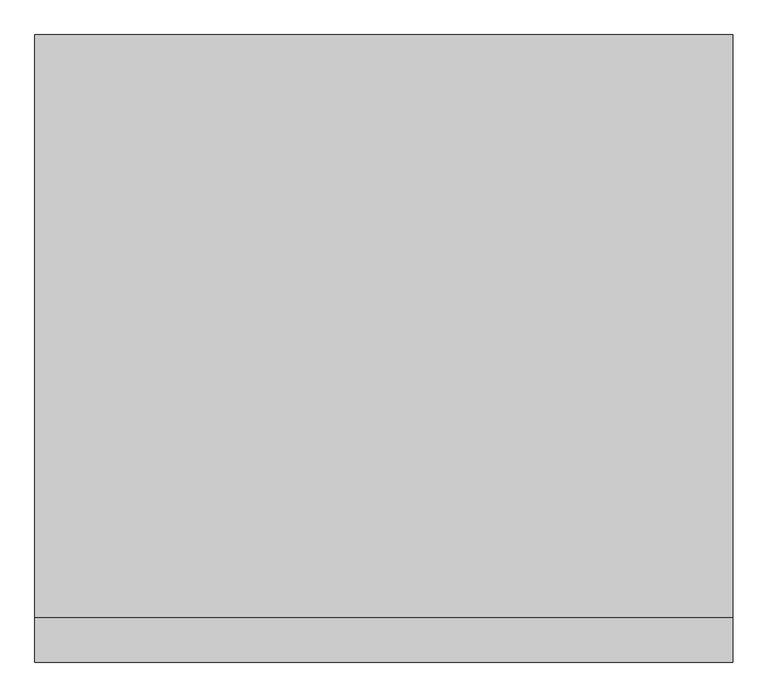
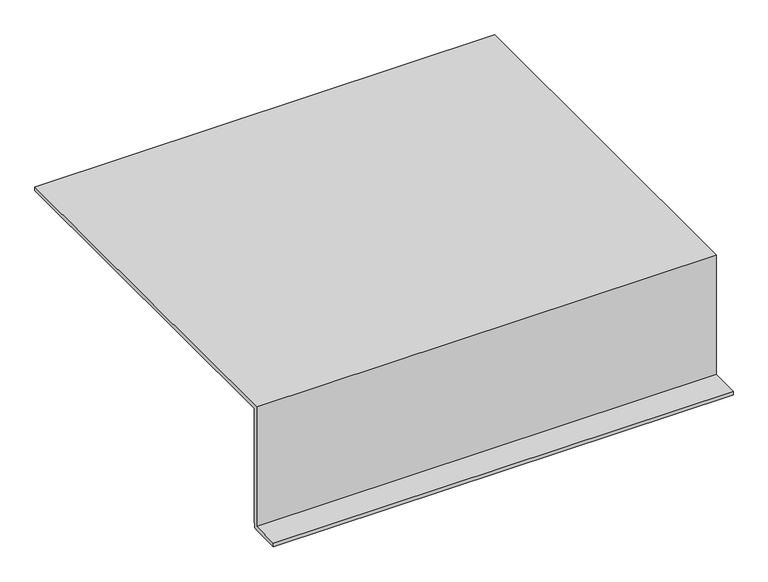
"""IFC4 building model written with IfcOpenShell, lengths in millimetres: proxy geometry, Gypsum020 5257 : Gypsum020 5257."""

from ifc_helpers import new_model, si_unit, frame, origin, place, context, project, spatial, polyline, outline, extrude, source, transform, mapped, element, save


def generic_models_33ea2bcf(model_context):
    return source(origin(), model_context, "Body", "SweptSolid", [
        extrude(outline(polyline([(-2827.7925368, 39553.8960938), (-4481.9675368, 39553.8960938), (-4481.9675368, 39025.6541813), (-4483.2475368, 39025.6541813), (-4483.2475368, 39004.5009974), (-4504.4007207, 39004.5009974), (-4504.4007207, 39003.2209974), (-4625.5194659, 39003.2209974), (-4625.5194659, 39019.0959974), (-4497.8424805, 39019.0959974), (-4497.8424805, 39569.7710938), (-2827.7925368, 39569.7710938), (-2827.7925368, 39553.8960938)])), frame((12383.0178845, 0.0, 0.0), z_axis=(1.0, 0.0, 0.0), x_axis=(0.0, 1.0, 0.0)), (0.0, 0.0, 1.0), 2000.0),
    ])


if __name__ == "__main__":
    model = new_model("IFC4")
    model_context = context("Model", 3, world=origin())
    ifc_project = project(units=[si_unit("LENGTHUNIT", "METRE", prefix="MILLI")], contexts=[model_context])
    site = spatial("IfcSite", under=ifc_project)
    building = spatial("IfcBuilding", under=site)
    placement = place(None, origin())
    generic_models_shape = generic_models_33ea2bcf(model_context)
    element("IfcBuildingElementProxy", 1, Name="Gypsum020 5257 : Gypsum020 5257", ObjectType="Gypsum020 5257 : Gypsum020 5257", at=placement, inside=building, context=model_context, shape_type="MappedRepresentation", body=[
        mapped(generic_models_shape, transform((0.0, 0.0, 0.0), x_axis=(1.0, 0.0, 0.0), y_axis=(0.0, 1.0, 0.0), z_axis=(0.0, 0.0, 1.0))),
    ])
    save(model, "model.ifc")

# Revit data of these elements
# Type "Gypsum020 5257 : Gypsum020 5257"
#   NameOverride = "Gypsum020"
# Element 1 (IfcBuildingElementProxy, "Gypsum020 5257 : Gypsum020 5257")
#   Materials on its faces: "5/8\" GYPSUM BOARD"
# Materials
#   "5/8\" GYPSUM BOARD": class "Unassigned", colour RGB 214 214 214, transparency 0, Cost = 0
